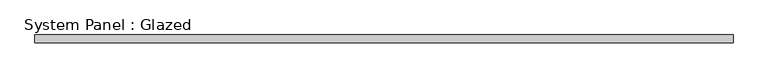
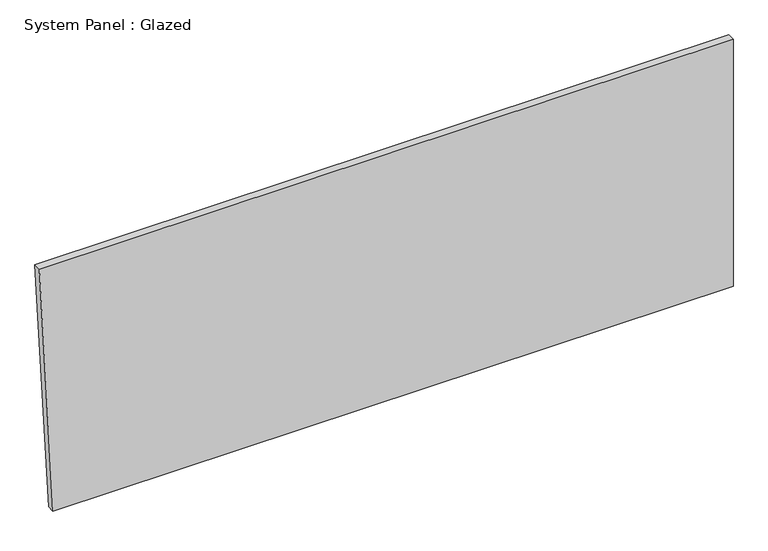
"""IFC4 building model written with IfcOpenShell, lengths in millimetres: plate geometry, System Panel : Glazed."""

import ifcopenshell
import ifcopenshell.guid

model = None  # the IFC model being written
_history = None  # IfcOwnerHistory: only IFC2X3 demands one
_inside = {}  # id of a spatial element -> (the spatial element, [elements in it])
_under = {}  # id of a project, library or spatial element -> (it, [spatial elements below it])
_declared = {}  # id of a project -> (the project, [libraries it declares])
_typed = {}  # id of a type object -> (the type object, [elements of that type])
_made_of = {}  # id of a material, layer set ... -> (it, [elements and type objects made of it])


def new_model(schema):
    """Start an empty IFC model of exactly this schema.

    Asked for "IFC4X3", IfcOpenShell would pick the latest addendum, in which some entities
    have other attributes; the version numbers below select the first issue.
    IFC2X3 requires an IfcOwnerHistory on every rooted entity: one is made here for all.
    """
    global model, _history
    if schema == "IFC4X3":
        model = ifcopenshell.file(schema_version=(4, 3, 0, 0))
    else:
        model = ifcopenshell.file(schema=schema)
    _inside.clear()
    _under.clear()
    _declared.clear()
    _typed.clear()
    _made_of.clear()
    _history = None
    if model.schema == "IFC2X3":
        org = make("IfcOrganization", Name="unknown")
        user = make(
            "IfcPersonAndOrganization",
            ThePerson=make("IfcPerson", FamilyName="unknown"),
            TheOrganization=org,
        )
        app = make(
            "IfcApplication",
            ApplicationDeveloper=org,
            Version="unknown",
            ApplicationFullName="unknown",
            ApplicationIdentifier="unknown",
        )
        _history = make(
            "IfcOwnerHistory",
            OwningUser=user,
            OwningApplication=app,
            ChangeAction="ADDED",
            CreationDate=0,
        )
    return model


def make(cls, **values):
    """One entity of the class cls with the attributes given. An attribute that is None is left unset."""
    return model.create_entity(
        cls, **{name: value for name, value in values.items() if value is not None}
    )


def rooted(cls, **values):
    """An entity with a GlobalId (a new one), such as an element, a storey or a relation."""
    return make(cls, GlobalId=ifcopenshell.guid.new(), OwnerHistory=_history, **values)


def si_unit(unit_type, name, prefix=None):
    """IfcSIUnit, for example si_unit("LENGTHUNIT", "METRE", prefix="MILLI")."""
    return make("IfcSIUnit", UnitType=unit_type, Prefix=prefix, Name=name)


def assignment(units):
    """IfcUnitAssignment: the units of a project."""
    return None if units is None else make("IfcUnitAssignment", Units=units)


def point(xyz):
    """IfcCartesianPoint."""
    return None if xyz is None else make("IfcCartesianPoint", Coordinates=xyz)


def direction(xyz):
    """IfcDirection."""
    return None if xyz is None else make("IfcDirection", DirectionRatios=xyz)


def frame(location, z_axis=None, x_axis=None):
    """IfcAxis2Placement3D, a coordinate frame: its origin and axes. An axis left out is left unset."""
    return make(
        "IfcAxis2Placement3D",
        Location=point(location),
        Axis=direction(z_axis),
        RefDirection=direction(x_axis),
    )


def origin():
    """The frame at (0, 0, 0) with its axes left unset."""
    return frame((0.0, 0.0, 0.0))


def place(relative_to, where):
    """IfcLocalPlacement: puts the frame where relative to a parent placement (None: the world)."""
    return make(
        "IfcLocalPlacement", PlacementRelTo=relative_to, RelativePlacement=where
    )


def context(
    kind, dimensions, precision=None, world=None, true_north=None, identifier=None
):
    """IfcGeometricRepresentationContext, for example the 3D "Model" context."""
    return make(
        "IfcGeometricRepresentationContext",
        ContextIdentifier=identifier,
        ContextType=kind,
        CoordinateSpaceDimension=dimensions,
        Precision=precision,
        WorldCoordinateSystem=world,
        TrueNorth=true_north,
    )


def project(units=None, contexts=None):
    """IfcProject with its units and contexts."""
    return rooted(
        "IfcProject",
        Name="project",
        RepresentationContexts=contexts,
        UnitsInContext=assignment(units),
    )


def spatial(cls, under=None, at=None, **own):
    """A site, building, storey or space (cls), placed at a placement, below another one or the project."""
    s = rooted(cls, ObjectPlacement=at, **own)
    if under is not None:
        _under.setdefault(under.id(), (under, []))[1].append(s)
    return s


def polyline(points):
    """IfcPolyline through the points."""
    return make("IfcPolyline", Points=[point(p) for p in points])


def outline(outer, holes=None, kind="AREA"):
    """IfcArbitraryClosedProfileDef: a profile drawn as a closed curve; with holes, ...WithVoids."""
    if holes is None:
        return make("IfcArbitraryClosedProfileDef", ProfileType=kind, OuterCurve=outer)
    return make(
        "IfcArbitraryProfileDefWithVoids",
        ProfileType=kind,
        OuterCurve=outer,
        InnerCurves=holes,
    )


def extrude(swept, where, along, depth):
    """IfcExtrudedAreaSolid: the profile swept, set in the frame where, extruded along a direction by depth."""
    return make(
        "IfcExtrudedAreaSolid",
        SweptArea=swept,
        Position=where,
        ExtrudedDirection=direction(along),
        Depth=depth,
    )


def shape(context_of_items, identifier, shape_type, items):
    """IfcShapeRepresentation: the items that make up one representation, for example the "Body"."""
    return make(
        "IfcShapeRepresentation",
        ContextOfItems=context_of_items,
        RepresentationIdentifier=identifier,
        RepresentationType=shape_type,
        Items=items,
    )


def source(mapping_origin, context_of_items, identifier, shape_type, items):
    """IfcRepresentationMap: a shape defined once, which mapped items show again and again."""
    return make(
        "IfcRepresentationMap",
        MappingOrigin=mapping_origin,
        MappedRepresentation=shape(context_of_items, identifier, shape_type, items),
    )


def transform(
    local_origin,
    x_axis=None,
    y_axis=None,
    z_axis=None,
    scale=None,
    scale2=None,
    scale3=None,
    uniform=True,
):
    """IfcCartesianTransformationOperator3D, or its non-uniform kind. x_axis, y_axis, z_axis: its Axis1, 2, 3."""
    if uniform:
        return make(
            "IfcCartesianTransformationOperator3D",
            Axis1=direction(x_axis),
            Axis2=direction(y_axis),
            LocalOrigin=point(local_origin),
            Scale=scale,
            Axis3=direction(z_axis),
        )
    return make(
        "IfcCartesianTransformationOperator3DnonUniform",
        Axis1=direction(x_axis),
        Axis2=direction(y_axis),
        LocalOrigin=point(local_origin),
        Scale=scale,
        Axis3=direction(z_axis),
        Scale2=scale2,
        Scale3=scale3,
    )


def mapped(mapping_source, mapping_target):
    """IfcMappedItem: shows the shape of a source again, moved by a transform."""
    return make(
        "IfcMappedItem", MappingSource=mapping_source, MappingTarget=mapping_target
    )


def made_of(thing, what):
    """Note that an element or type object is made of a material, layer set ...; save() writes the relation."""
    if what is not None:
        _made_of.setdefault(what.id(), (what, []))[1].append(thing)
    return thing


def element(
    cls,
    number,
    at=None,
    inside=None,
    cuts=None,
    type_object=None,
    material=None,
    context=None,
    identifier="Body",
    shape_type=None,
    held_by="IfcProductDefinitionShape",
    body=None,
    shapes=None,
    **own,
):
    """One element of the class cls, such as IfcWall. Its Tag is "e" and its number.

    at: its placement. inside: the storey or other place that contains it. cuts: it is an
    opening in that element (IfcRelVoidsElement). A single representation is given by context,
    identifier, shape_type and body (its items); several are given by shapes. held_by: the class
    of the entity that holds the representations. save() writes the other relations.
    """
    e = rooted(cls, Tag="e%d" % number, ObjectPlacement=at, **own)
    if body is not None:
        shapes = [shape(context, identifier, shape_type, body)]
    if shapes is not None:
        e.Representation = make(held_by, Representations=shapes)
    if inside is not None:
        _inside.setdefault(inside.id(), (inside, []))[1].append(e)
    if cuts is not None:
        rooted(
            "IfcRelVoidsElement", RelatingBuildingElement=cuts, RelatedOpeningElement=e
        )
    if type_object is not None:
        _typed.setdefault(type_object.id(), (type_object, []))[1].append(e)
    return made_of(e, material)


def aggregate(whole, parts):
    """IfcRelAggregates: a whole, such as a stair, and the parts it consists of."""
    return rooted("IfcRelAggregates", RelatingObject=whole, RelatedObjects=parts)


def save(model, path):
    """Write the relations noted so far, then the file.

    IfcRelAggregates (storeys below a building ...), IfcRelContainedInSpatialStructure (elements
    in a storey), IfcRelDefinesByType, IfcRelAssociatesMaterial and IfcRelDeclares: one each for
    every whole, place, type object, material and project.
    """
    for whole, parts in _under.values():
        aggregate(whole, parts)
    for where, things in _inside.values():
        rooted(
            "IfcRelContainedInSpatialStructure",
            RelatedElements=things,
            RelatingStructure=where,
        )
    for kind, things in _typed.values():
        rooted("IfcRelDefinesByType", RelatedObjects=things, RelatingType=kind)
    for what, things in _made_of.values():
        rooted("IfcRelAssociatesMaterial", RelatedObjects=things, RelatingMaterial=what)
    for by, libraries in _declared.values():
        rooted("IfcRelDeclares", RelatingContext=by, RelatedDefinitions=libraries)
    model.write(path)


def system_panel_glazed_624ae8a5(model_context):
    return source(origin(), model_context, "Body", "SweptSolid", [
        extrude(outline(polyline([(0.0, -1106.180401), (0.0, 1151.5076076), (866.081558, 1151.5076076), (866.081558, -1151.5076076), (0.0, -1106.180401)])), frame((0.0, -44.45, 0.0), z_axis=(0.0, 1.0, 0.0), x_axis=(0.0, 0.0, 1.0)), (0.0, 0.0, 1.0), 25.4),
    ])


if __name__ == "__main__":
    model = new_model("IFC4")
    model_context = context("Model", 3, world=origin())
    ifc_project = project(units=[si_unit("LENGTHUNIT", "METRE", prefix="MILLI")], contexts=[model_context])
    site = spatial("IfcSite", under=ifc_project)
    building = spatial("IfcBuilding", under=site)
    placement = place(None, origin())
    system_panel_glazed_shape = system_panel_glazed_624ae8a5(model_context)
    element("IfcPlate", 1, ObjectType="System Panel : Glazed", at=placement, inside=building, context=model_context, shape_type="MappedRepresentation", body=[
        mapped(system_panel_glazed_shape, transform((0.0, 0.0, 0.0), x_axis=(1.0, 0.0, 0.0), y_axis=(0.0, 1.0, 0.0), z_axis=(0.0, 0.0, 1.0))),
    ])
    save(model, "model.ifc")

# Revit data of these elements
# Type "System Panel : Glazed"
#   Construction Type Id = "GSP4R"
#   Analytic Construction = "1/8 in Pilkington single glazing"
#   Visual Light Transmittance = 0.9
#   Solar Heat Gain Coefficient = 0.86
#   Heat Transfer Coefficient (U) = 1.18115 BTU/(h·ft²·°F)
#   Define Thermal Properties by = 1
# Element 1 (IfcPlate, "System Panel : Glazed")
#   Materials on its faces: "Glass"
# Materials
#   "Glass": class "Glass", colour RGB 0 128 192, transparency 0.75, Description = "Soda Lime Glass", Cost = 0
